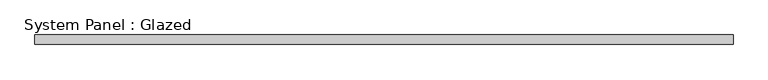
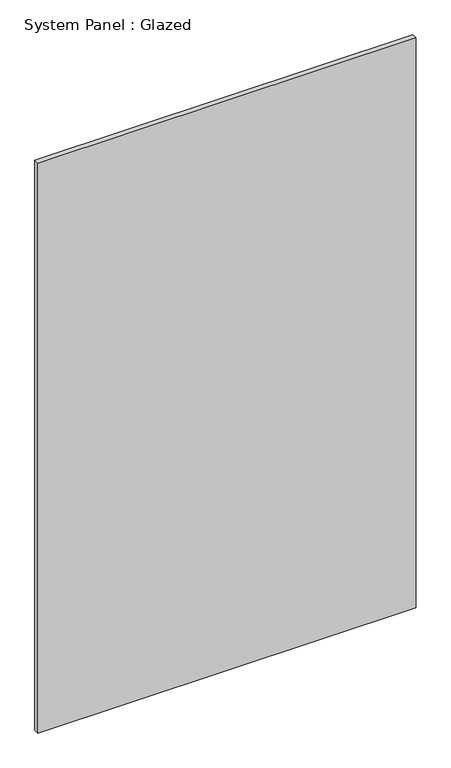
"""IFC4 building model written with IfcOpenShell, lengths in millimetres: plate geometry, System Panel : Glazed."""

from ifc_helpers import new_model, si_unit, origin, origin_with_axes, place, context, project, spatial, polyline, outline, extrude, source, transform, mapped, element, save


def system_panel_glazed_2c2a58be(model_context):
    return source(origin(), model_context, "Body", "SweptSolid", [
        extrude(outline(polyline([(918.0833333, 24.5), (-918.0833333, 24.5), (-918.0833333, 49.5), (918.0833333, 49.5), (918.0833333, 24.5)])), origin_with_axes(), (0.0, 0.0, 1.0), 2925.0),
    ])


if __name__ == "__main__":
    model = new_model("IFC4")
    model_context = context("Model", 3, world=origin())
    ifc_project = project(units=[si_unit("LENGTHUNIT", "METRE", prefix="MILLI")], contexts=[model_context])
    site = spatial("IfcSite", under=ifc_project)
    building = spatial("IfcBuilding", under=site)
    placement = place(None, origin())
    system_panel_glazed_shape = system_panel_glazed_2c2a58be(model_context)
    element("IfcPlate", 1, ObjectType="System Panel : Glazed", at=placement, inside=building, context=model_context, shape_type="MappedRepresentation", body=[
        mapped(system_panel_glazed_shape, transform((0.0, 0.0, 0.0), x_axis=(1.0, 0.0, 0.0), y_axis=(0.0, 1.0, 0.0), z_axis=(0.0, 0.0, 1.0))),
    ])
    save(model, "model.ifc")

# Revit data of these elements
# Element 1 (IfcPlate, "System Panel : Glazed")
#   Materials on its faces: "Glass"
# Materials
#   "Glass": class "Glass", colour RGB 0 128 192, transparency 0.9
